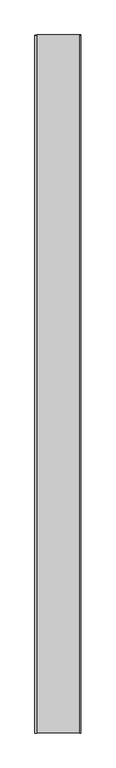
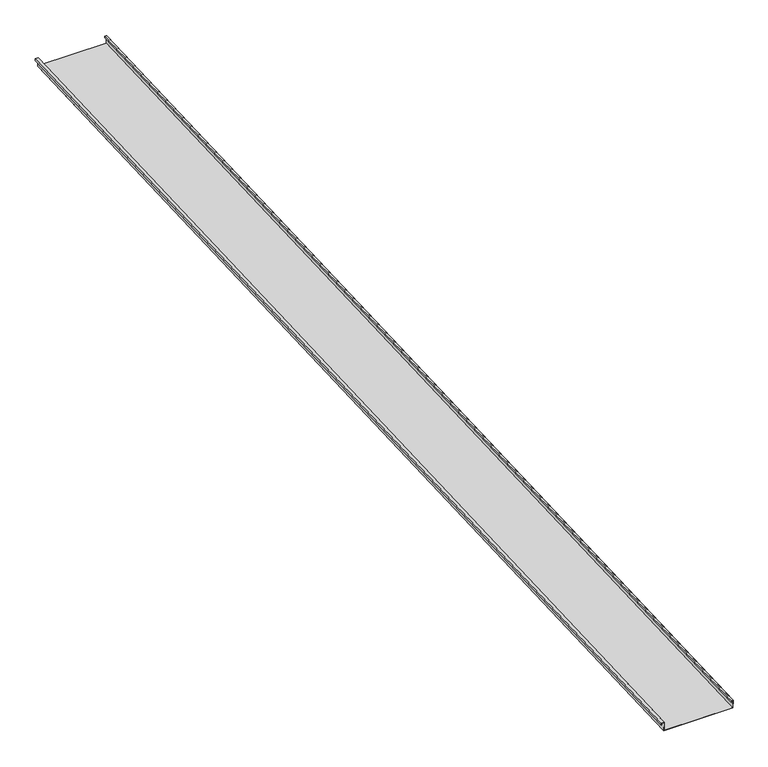
"""IFC4 building model written with IfcOpenShell, lengths in millimetres: proxy geometry, Generic Models 2:Generic Models 2:310765:Generic Models 2:310765 : Generic Models 2:Generic Models 2:310765:117 : Generic Models 2:Generic Models 2:310765:Generic Models 2:310765 : Generic Models 2:Generic Models 2:310765:300385."""

from ifc_helpers import new_model, si_unit, frame, origin, place, context, project, spatial, polyline, outline, extrude, source, transform, mapped, element, save


def generic_models_6cb5c50d(model_context):
    return source(origin(), model_context, "Body", "SweptSolid", [
        extrude(outline(polyline([(1.5875, 0.0), (1.5875, 50.8), (407.9875, 50.8), (407.9875, 1.5875), (396.875, 1.5875), (396.875, 11.1125), (398.4625, 11.1125), (398.4625, 3.175), (406.4, 3.175), (406.4, 49.2125), (3.175, 49.2125), (3.175, -1.5874999), (-14.2875, -1.5874999), (-14.2875, 9.525), (-12.7, 9.525), (-12.7, 0.0), (1.5875, 0.0)])), frame((665026.6263072, -581354.4345603, 3902.6697972), z_axis=(0.0, 0.9991330730923568, 0.041630544712067834), x_axis=(1.0, 0.0, 0.0)), (0.0, 0.0, 1.0), 6400.8),
    ])


if __name__ == "__main__":
    model = new_model("IFC4")
    model_context = context("Model", 3, world=origin())
    ifc_project = project(units=[si_unit("LENGTHUNIT", "METRE", prefix="MILLI")], contexts=[model_context])
    site = spatial("IfcSite", under=ifc_project)
    building = spatial("IfcBuilding", under=site)
    placement = place(None, origin())
    generic_models_shape = generic_models_6cb5c50d(model_context)
    element("IfcBuildingElementProxy", 1, Name="Generic Models 2:Generic Models 2:310765:Generic Models 2:310765 : Generic Models 2:Generic Models 2:310765:117 : Generic Models 2:Generic Models 2:310765:Generic Models 2:310765 : Generic Models 2:Generic Models 2:310765:300385", ObjectType="Generic Models 2:Generic Models 2:310765:Generic Models 2:310765 : Generic Models 2:Generic Models 2:310765:117 : Generic Models 2:Generic Models 2:310765:Generic Models 2:310765 : Generic Models 2:Generic Models 2:310765:300385", at=placement, inside=building, context=model_context, shape_type="MappedRepresentation", body=[
        mapped(generic_models_shape, transform((0.0, 0.0, 0.0), x_axis=(1.0, 0.0, 0.0), y_axis=(0.0, 1.0, 0.0), z_axis=(0.0, 0.0, 1.0))),
    ])
    save(model, "model.ifc")

# Revit data of these elements
# Type "Generic Models 2:Generic Models 2:310765:Generic Models 2:310765 : Generic Models 2:Generic Models 2:310765:117 : Generic Models 2:Generic Models 2:310765:Generic Models 2:310765 : Generic Models 2:Generic Models 2:310765:300385"
#   NameOverride = "Generic Models 2:Generic Models 2:310765:Generic Models 2:310765 : Generic Models 2:Generic Models 2:310765:300385"
#   ObjectTypeOverride = "Generic Models 2:310765 : Generic Models 2:Generic Models 2:310765"
#   Reference = "Generic Models 2"
#   Tag = "300385"
# Element 1 (IfcBuildingElementProxy, "Generic Models 2:Generic Models 2:310765:Generic Models 2:310765 : Generic Models 2:Generic Models 2:310765:117 : Generic Models 2:Generic Models 2:310765:Generic Models 2:310765 : Generic Models 2:Generic Models 2:310765:300385")
#   Materials on its faces: "THERMAL BROKEN ALUMINUM STOREFRONT FOR POLYCARBONATE"
# Materials
#   "THERMAL BROKEN ALUMINUM STOREFRONT FOR POLYCARBONATE": class "Unassigned", colour RGB 244 244 244, transparency 0, Keynote = "M07611300.01", Cost = 0
